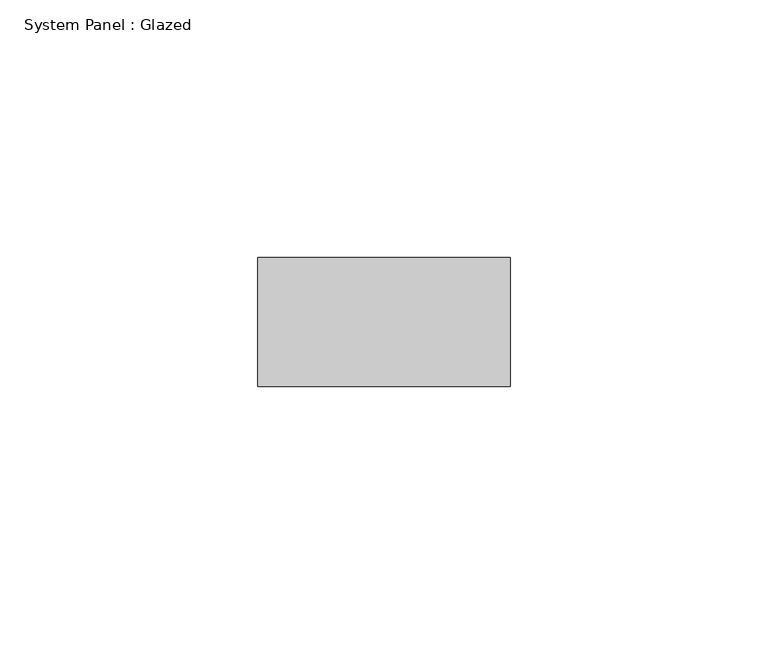
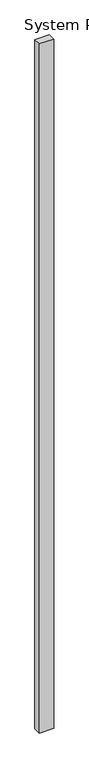
"""IFC4 building model written with IfcOpenShell, lengths in millimetres: plate geometry, System Panel : Glazed."""

from ifc_helpers import new_model, si_unit, origin, origin_with_axes, place, context, project, spatial, polyline, outline, extrude, source, transform, mapped, element, save


def system_panel_glazed_867a6306(model_context):
    return source(origin(), model_context, "Body", "SweptSolid", [
        extrude(outline(polyline([(24.5092572, -49.5), (-24.5092572, -49.5), (-24.5092572, -24.5), (24.5092572, -24.5), (24.5092572, -49.5)])), origin_with_axes(), (0.0, 0.0, 1.0), 2450.0),
    ])


if __name__ == "__main__":
    model = new_model("IFC4")
    model_context = context("Model", 3, world=origin())
    ifc_project = project(units=[si_unit("LENGTHUNIT", "METRE", prefix="MILLI")], contexts=[model_context])
    site = spatial("IfcSite", under=ifc_project)
    building = spatial("IfcBuilding", under=site)
    placement = place(None, origin())
    system_panel_glazed_shape = system_panel_glazed_867a6306(model_context)
    element("IfcPlate", 1, ObjectType="System Panel : Glazed", at=placement, inside=building, context=model_context, shape_type="MappedRepresentation", body=[
        mapped(system_panel_glazed_shape, transform((0.0, 0.0, 0.0), x_axis=(1.0, 0.0, 0.0), y_axis=(0.0, 1.0, 0.0), z_axis=(0.0, 0.0, 1.0))),
    ])
    save(model, "model.ifc")

# Revit data of these elements
# Type "System Panel : Glazed"
#   Keynote = "H11"
#   Construction Type Id = "GSP4R"
#   Analytic Construction = "1/8 in Pilkington single glazing"
#   Visual Light Transmittance = 0.9
#   Solar Heat Gain Coefficient = 0.86
#   Heat Transfer Coefficient (U) = 6.7069 W/(m²·K)
# Element 1 (IfcPlate, "System Panel : Glazed")
#   Materials on its faces: "Glass"
# Materials
#   "Glass": class "Glass", colour RGB 0 128 192, transparency 0.9, Description = "Soda Lime Glass", Cost = 0
